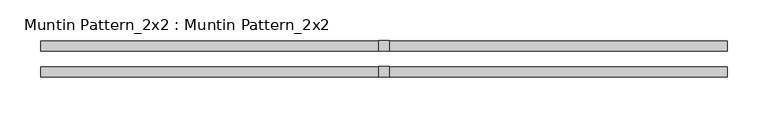
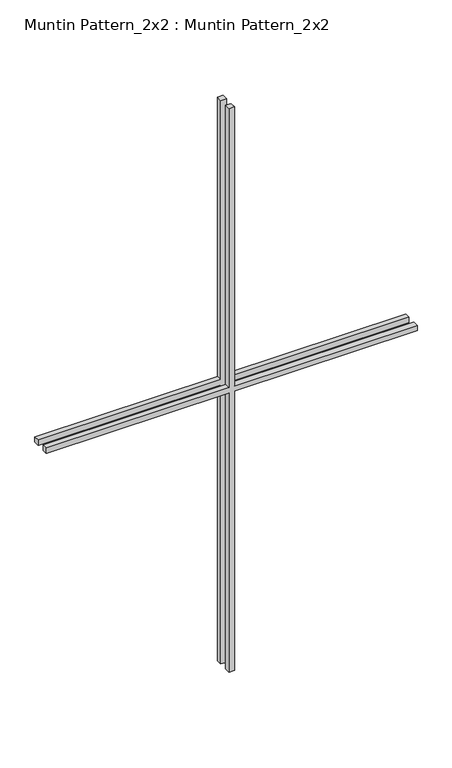
"""IFC4 building model written with IfcOpenShell, lengths in millimetres: proxy geometry, Muntin Pattern_2x2 : Muntin Pattern_2x2."""

import ifcopenshell
import ifcopenshell.guid

model = None  # the IFC model being written
_history = None  # IfcOwnerHistory: only IFC2X3 demands one
_inside = {}  # id of a spatial element -> (the spatial element, [elements in it])
_under = {}  # id of a project, library or spatial element -> (it, [spatial elements below it])
_declared = {}  # id of a project -> (the project, [libraries it declares])
_typed = {}  # id of a type object -> (the type object, [elements of that type])
_made_of = {}  # id of a material, layer set ... -> (it, [elements and type objects made of it])


def new_model(schema):
    """Start an empty IFC model of exactly this schema.

    Asked for "IFC4X3", IfcOpenShell would pick the latest addendum, in which some entities
    have other attributes; the version numbers below select the first issue.
    IFC2X3 requires an IfcOwnerHistory on every rooted entity: one is made here for all.
    """
    global model, _history
    if schema == "IFC4X3":
        model = ifcopenshell.file(schema_version=(4, 3, 0, 0))
    else:
        model = ifcopenshell.file(schema=schema)
    _inside.clear()
    _under.clear()
    _declared.clear()
    _typed.clear()
    _made_of.clear()
    _history = None
    if model.schema == "IFC2X3":
        org = make("IfcOrganization", Name="unknown")
        user = make(
            "IfcPersonAndOrganization",
            ThePerson=make("IfcPerson", FamilyName="unknown"),
            TheOrganization=org,
        )
        app = make(
            "IfcApplication",
            ApplicationDeveloper=org,
            Version="unknown",
            ApplicationFullName="unknown",
            ApplicationIdentifier="unknown",
        )
        _history = make(
            "IfcOwnerHistory",
            OwningUser=user,
            OwningApplication=app,
            ChangeAction="ADDED",
            CreationDate=0,
        )
    return model


def make(cls, **values):
    """One entity of the class cls with the attributes given. An attribute that is None is left unset."""
    return model.create_entity(
        cls, **{name: value for name, value in values.items() if value is not None}
    )


def rooted(cls, **values):
    """An entity with a GlobalId (a new one), such as an element, a storey or a relation."""
    return make(cls, GlobalId=ifcopenshell.guid.new(), OwnerHistory=_history, **values)


def si_unit(unit_type, name, prefix=None):
    """IfcSIUnit, for example si_unit("LENGTHUNIT", "METRE", prefix="MILLI")."""
    return make("IfcSIUnit", UnitType=unit_type, Prefix=prefix, Name=name)


def assignment(units):
    """IfcUnitAssignment: the units of a project."""
    return None if units is None else make("IfcUnitAssignment", Units=units)


def point(xyz):
    """IfcCartesianPoint."""
    return None if xyz is None else make("IfcCartesianPoint", Coordinates=xyz)


def direction(xyz):
    """IfcDirection."""
    return None if xyz is None else make("IfcDirection", DirectionRatios=xyz)


def frame(location, z_axis=None, x_axis=None):
    """IfcAxis2Placement3D, a coordinate frame: its origin and axes. An axis left out is left unset."""
    return make(
        "IfcAxis2Placement3D",
        Location=point(location),
        Axis=direction(z_axis),
        RefDirection=direction(x_axis),
    )


def origin():
    """The frame at (0, 0, 0) with its axes left unset."""
    return frame((0.0, 0.0, 0.0))


def place(relative_to, where):
    """IfcLocalPlacement: puts the frame where relative to a parent placement (None: the world)."""
    return make(
        "IfcLocalPlacement", PlacementRelTo=relative_to, RelativePlacement=where
    )


def context(
    kind, dimensions, precision=None, world=None, true_north=None, identifier=None
):
    """IfcGeometricRepresentationContext, for example the 3D "Model" context."""
    return make(
        "IfcGeometricRepresentationContext",
        ContextIdentifier=identifier,
        ContextType=kind,
        CoordinateSpaceDimension=dimensions,
        Precision=precision,
        WorldCoordinateSystem=world,
        TrueNorth=true_north,
    )


def project(units=None, contexts=None):
    """IfcProject with its units and contexts."""
    return rooted(
        "IfcProject",
        Name="project",
        RepresentationContexts=contexts,
        UnitsInContext=assignment(units),
    )


def spatial(cls, under=None, at=None, **own):
    """A site, building, storey or space (cls), placed at a placement, below another one or the project."""
    s = rooted(cls, ObjectPlacement=at, **own)
    if under is not None:
        _under.setdefault(under.id(), (under, []))[1].append(s)
    return s


def polyline(points):
    """IfcPolyline through the points."""
    return make("IfcPolyline", Points=[point(p) for p in points])


def outline(outer, holes=None, kind="AREA"):
    """IfcArbitraryClosedProfileDef: a profile drawn as a closed curve; with holes, ...WithVoids."""
    if holes is None:
        return make("IfcArbitraryClosedProfileDef", ProfileType=kind, OuterCurve=outer)
    return make(
        "IfcArbitraryProfileDefWithVoids",
        ProfileType=kind,
        OuterCurve=outer,
        InnerCurves=holes,
    )


def extrude(swept, where, along, depth):
    """IfcExtrudedAreaSolid: the profile swept, set in the frame where, extruded along a direction by depth."""
    return make(
        "IfcExtrudedAreaSolid",
        SweptArea=swept,
        Position=where,
        ExtrudedDirection=direction(along),
        Depth=depth,
    )


def shape(context_of_items, identifier, shape_type, items):
    """IfcShapeRepresentation: the items that make up one representation, for example the "Body"."""
    return make(
        "IfcShapeRepresentation",
        ContextOfItems=context_of_items,
        RepresentationIdentifier=identifier,
        RepresentationType=shape_type,
        Items=items,
    )


def source(mapping_origin, context_of_items, identifier, shape_type, items):
    """IfcRepresentationMap: a shape defined once, which mapped items show again and again."""
    return make(
        "IfcRepresentationMap",
        MappingOrigin=mapping_origin,
        MappedRepresentation=shape(context_of_items, identifier, shape_type, items),
    )


def transform(
    local_origin,
    x_axis=None,
    y_axis=None,
    z_axis=None,
    scale=None,
    scale2=None,
    scale3=None,
    uniform=True,
):
    """IfcCartesianTransformationOperator3D, or its non-uniform kind. x_axis, y_axis, z_axis: its Axis1, 2, 3."""
    if uniform:
        return make(
            "IfcCartesianTransformationOperator3D",
            Axis1=direction(x_axis),
            Axis2=direction(y_axis),
            LocalOrigin=point(local_origin),
            Scale=scale,
            Axis3=direction(z_axis),
        )
    return make(
        "IfcCartesianTransformationOperator3DnonUniform",
        Axis1=direction(x_axis),
        Axis2=direction(y_axis),
        LocalOrigin=point(local_origin),
        Scale=scale,
        Axis3=direction(z_axis),
        Scale2=scale2,
        Scale3=scale3,
    )


def mapped(mapping_source, mapping_target):
    """IfcMappedItem: shows the shape of a source again, moved by a transform."""
    return make(
        "IfcMappedItem", MappingSource=mapping_source, MappingTarget=mapping_target
    )


def made_of(thing, what):
    """Note that an element or type object is made of a material, layer set ...; save() writes the relation."""
    if what is not None:
        _made_of.setdefault(what.id(), (what, []))[1].append(thing)
    return thing


def element(
    cls,
    number,
    at=None,
    inside=None,
    cuts=None,
    type_object=None,
    material=None,
    context=None,
    identifier="Body",
    shape_type=None,
    held_by="IfcProductDefinitionShape",
    body=None,
    shapes=None,
    **own,
):
    """One element of the class cls, such as IfcWall. Its Tag is "e" and its number.

    at: its placement. inside: the storey or other place that contains it. cuts: it is an
    opening in that element (IfcRelVoidsElement). A single representation is given by context,
    identifier, shape_type and body (its items); several are given by shapes. held_by: the class
    of the entity that holds the representations. save() writes the other relations.
    """
    e = rooted(cls, Tag="e%d" % number, ObjectPlacement=at, **own)
    if body is not None:
        shapes = [shape(context, identifier, shape_type, body)]
    if shapes is not None:
        e.Representation = make(held_by, Representations=shapes)
    if inside is not None:
        _inside.setdefault(inside.id(), (inside, []))[1].append(e)
    if cuts is not None:
        rooted(
            "IfcRelVoidsElement", RelatingBuildingElement=cuts, RelatedOpeningElement=e
        )
    if type_object is not None:
        _typed.setdefault(type_object.id(), (type_object, []))[1].append(e)
    return made_of(e, material)


def aggregate(whole, parts):
    """IfcRelAggregates: a whole, such as a stair, and the parts it consists of."""
    return rooted("IfcRelAggregates", RelatingObject=whole, RelatedObjects=parts)


def save(model, path):
    """Write the relations noted so far, then the file.

    IfcRelAggregates (storeys below a building ...), IfcRelContainedInSpatialStructure (elements
    in a storey), IfcRelDefinesByType, IfcRelAssociatesMaterial and IfcRelDeclares: one each for
    every whole, place, type object, material and project.
    """
    for whole, parts in _under.values():
        aggregate(whole, parts)
    for where, things in _inside.values():
        rooted(
            "IfcRelContainedInSpatialStructure",
            RelatedElements=things,
            RelatingStructure=where,
        )
    for kind, things in _typed.values():
        rooted("IfcRelDefinesByType", RelatedObjects=things, RelatingType=kind)
    for what, things in _made_of.values():
        rooted("IfcRelAssociatesMaterial", RelatedObjects=things, RelatingMaterial=what)
    for by, libraries in _declared.values():
        rooted("IfcRelDeclares", RelatingContext=by, RelatedDefinitions=libraries)
    model.write(path)


def muntin_pattern_2x2_muntin_pattern_2x2_809937e0(model_context):
    return source(origin(), model_context, "Body", "SweptSolid", [
        extrude(outline(polyline([(679.45, -6.35), (679.45, -419.1), (666.75, -419.1), (666.75, -6.35), (0.0, -6.35), (0.0, 6.35), (666.75, 6.35), (666.75, 419.1), (679.45, 419.1), (679.45, 6.35), (1346.2, 6.35), (1346.2, -6.35), (679.45, -6.35)])), frame((0.0, -22.225, 0.0), z_axis=(0.0, 1.0, 0.0), x_axis=(0.0, 0.0, 1.0)), (0.0, 0.0, 1.0), 12.7),
        extrude(outline(polyline([(679.45, -6.35), (679.45, -419.1), (666.75, -419.1), (666.75, -6.35), (0.0, -6.35), (0.0, 6.35), (666.75, 6.35), (666.75, 419.1), (679.45, 419.1), (679.45, 6.35), (1346.2, 6.35), (1346.2, -6.35), (679.45, -6.35)])), frame((0.0, 9.525, 0.0), z_axis=(0.0, 1.0, 0.0), x_axis=(0.0, 0.0, 1.0)), (0.0, 0.0, 1.0), 12.7),
    ])


if __name__ == "__main__":
    model = new_model("IFC4")
    model_context = context("Model", 3, world=origin())
    ifc_project = project(units=[si_unit("LENGTHUNIT", "METRE", prefix="MILLI")], contexts=[model_context])
    site = spatial("IfcSite", under=ifc_project)
    building = spatial("IfcBuilding", under=site)
    placement = place(None, origin())
    muntin_pattern_2x2_muntin_pattern_2x2_shape = muntin_pattern_2x2_muntin_pattern_2x2_809937e0(model_context)
    element("IfcBuildingElementProxy", 1, Name="Muntin Pattern_2x2 : Muntin Pattern_2x2", ObjectType="Muntin Pattern_2x2 : Muntin Pattern_2x2", at=placement, inside=building, context=model_context, shape_type="MappedRepresentation", body=[
        mapped(muntin_pattern_2x2_muntin_pattern_2x2_shape, transform((0.0, 0.0, 0.0), x_axis=(1.0, 0.0, 0.0), y_axis=(0.0, 1.0, 0.0), z_axis=(0.0, 0.0, 1.0))),
    ])
    save(model, "model.ifc")

# Revit data of these elements
# Type "Muntin Pattern_2x2 : Muntin Pattern_2x2"
#   Width [instance default] = 4' - 0"
#   Thickness = 0' - 0 1/2"
#   Height [instance default] = 4' - 0"
#   Distance = 0' - 0 3/4"
#   Interior Material [instance default] = none
#   Exterior Material [instance default] = none
#   Default Elevation = 0
# Element 1 (IfcBuildingElementProxy, "Muntin Pattern_2x2 : Muntin Pattern_2x2")
#   Width = 2' - 9"
#   Height = 4' - 5"
#   Interior Material = Wood - Stained
#   Exterior Material = Clad - White
#   Materials on its faces: "Clad - White", "Wood - Stained"
# Materials
#   "Clad - White": class "Wood", colour RGB 242 242 238, transparency 0, Cost = 0
#   "Wood - Stained": class "Wood", colour RGB 224 178 126, transparency 0, Cost = 0
